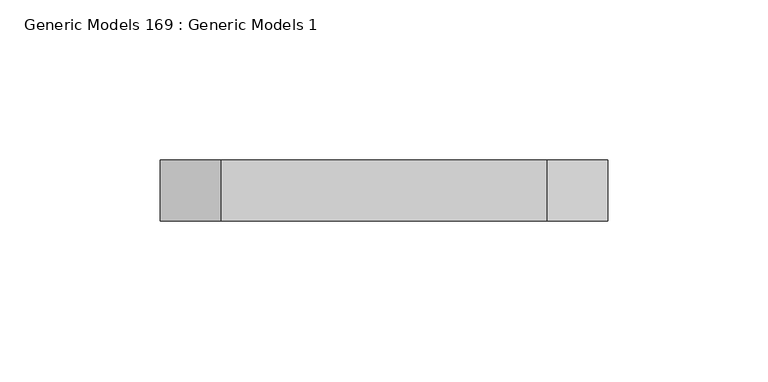
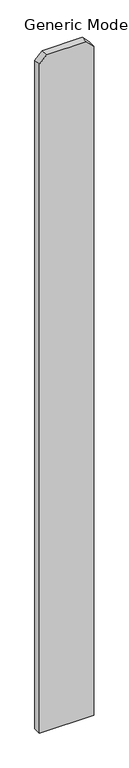
"""IFC4 building model written with IfcOpenShell, lengths in millimetres: proxy geometry, Generic Models 169 : Generic Models 1."""

from ifc_helpers import new_model, si_unit, frame, origin, place, context, project, spatial, polyline, outline, extrude, source, transform, mapped, element, save


def generic_models_169_generic_models_1_bddc7243(model_context):
    return source(origin(), model_context, "Body", "SweptSolid", [
        extrude(outline(polyline([(76.2, 55751.4125), (1885.95, 55751.4125), (1905.0, 55732.3625), (1905.0, 55630.7625), (1885.95, 55611.7125), (76.2, 55611.7125), (76.2, 55751.4125)])), frame((0.0, 547.6875, 0.0), z_axis=(0.0, 1.0, 0.0), x_axis=(0.0, 0.0, 1.0)), (0.0, 0.0, 1.0), 19.05),
    ])


if __name__ == "__main__":
    model = new_model("IFC4")
    model_context = context("Model", 3, world=origin())
    ifc_project = project(units=[si_unit("LENGTHUNIT", "METRE", prefix="MILLI")], contexts=[model_context])
    site = spatial("IfcSite", under=ifc_project)
    building = spatial("IfcBuilding", under=site)
    placement = place(None, origin())
    generic_models_169_generic_models_1_shape = generic_models_169_generic_models_1_bddc7243(model_context)
    element("IfcBuildingElementProxy", 1, Name="Generic Models 169 : Generic Models 1", ObjectType="Generic Models 169 : Generic Models 1", at=placement, inside=building, context=model_context, shape_type="MappedRepresentation", body=[
        mapped(generic_models_169_generic_models_1_shape, transform((0.0, 0.0, 0.0), x_axis=(1.0, 0.0, 0.0), y_axis=(0.0, 1.0, 0.0), z_axis=(0.0, 0.0, 1.0))),
    ])
    save(model, "model.ifc")

# Revit data of these elements
# Element 1 (IfcBuildingElementProxy, "Generic Models 169 : Generic Models 1")
#   Materials on its faces: "VERTICAL 1X6 CEDAR PLANKS W/ CLEAR WOOD SEALER"
# Materials
#   "VERTICAL 1X6 CEDAR PLANKS W/ CLEAR WOOD SEALER": class "Wood", colour RGB 234 198 147, transparency 0, Description = "Pinus Echinata", Cost = 0
